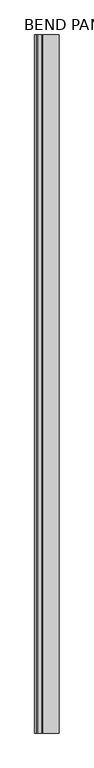
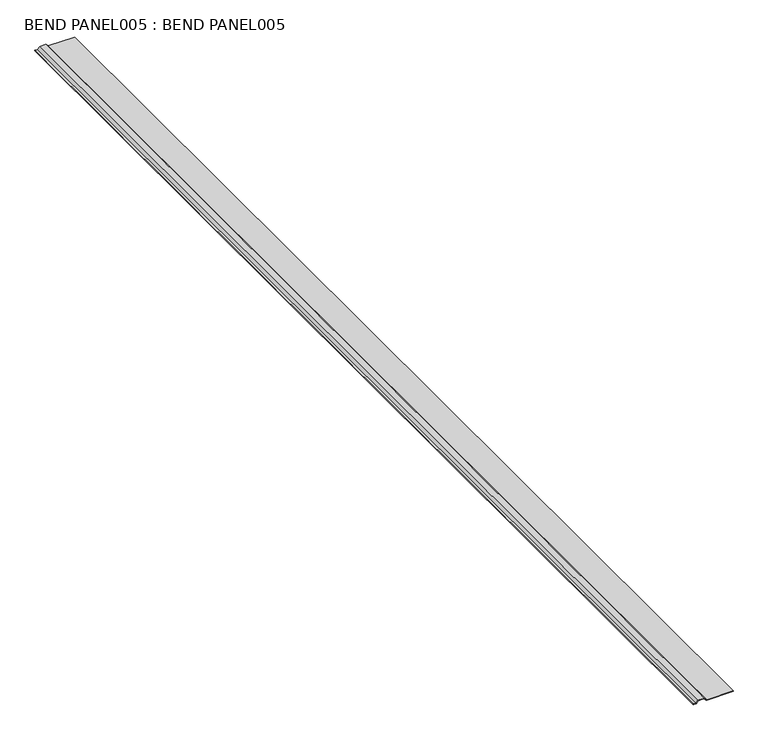
"""IFC4 building model written with IfcOpenShell, lengths in millimetres: proxy geometry, BEND PANEL005 : BEND PANEL005."""

from ifc_helpers import new_model, si_unit, point, frame, frame_2d, origin, place, context, project, spatial, polyline, circle_curve, trimmed, segment, composite_curve, outline, extrude, source, transform, mapped, element, save


def bend_panel005_bend_panel005_8c87a596(model_context):
    return source(origin(), model_context, "Body", "SweptSolid", [
        extrude(outline(composite_curve([segment(polyline([(42575.4212949, 5895.2230694), (42576.6119199, 5895.2230694), (42576.6119199, 5848.7155886), (42580.7948046, 5844.5327039), (42580.7948046, 5833.5642507), (42576.6119199, 5829.381366), (42576.6119199, 5825.5083246), (42575.4212949, 5825.5083246), (42575.4212949, 5829.381366)]), True, "CONTINUOUS"), segment(trimmed(circle_curve(frame_2d((42576.6119199, 5829.381366)), 1.190625), [point((42575.4212949, 5829.381366))], [point((42575.7700209, 5830.223265))], False, "CARTESIAN"), True, "CONTINUOUS"), segment(polyline([(42575.7700209, 5830.223265), (42579.6041796, 5834.0574237), (42579.6041796, 5844.0395308), (42575.7700209, 5847.8736895)]), True, "CONTINUOUS"), segment(trimmed(circle_curve(frame_2d((42576.6119199, 5848.7155885)), 1.190625), [point((42575.7700209, 5847.8736895))], [point((42575.4212949, 5848.7155885))], False, "CARTESIAN"), True, "CONTINUOUS"), segment(polyline([(42575.4212949, 5848.7155885), (42575.4212949, 5895.2230694)]), True, "CONTINUOUS")], self_intersect=False)), frame((0.0, -1052.8906574, 0.0), z_axis=(0.0, 1.0, 0.0), x_axis=(0.0, 0.0, 1.0)), (0.0, 0.0, 1.0), 1999.85),
    ])


if __name__ == "__main__":
    model = new_model("IFC4")
    model_context = context("Model", 3, world=origin())
    ifc_project = project(units=[si_unit("LENGTHUNIT", "METRE", prefix="MILLI")], contexts=[model_context])
    site = spatial("IfcSite", under=ifc_project)
    building = spatial("IfcBuilding", under=site)
    placement = place(None, origin())
    bend_panel005_bend_panel005_shape = bend_panel005_bend_panel005_8c87a596(model_context)
    element("IfcBuildingElementProxy", 1, Name="BEND PANEL005 : BEND PANEL005", ObjectType="BEND PANEL005 : BEND PANEL005", at=placement, inside=building, context=model_context, shape_type="MappedRepresentation", body=[
        mapped(bend_panel005_bend_panel005_shape, transform((0.0, 0.0, 0.0), x_axis=(1.0, 0.0, 0.0), y_axis=(0.0, 1.0, 0.0), z_axis=(0.0, 0.0, 1.0))),
    ])
    save(model, "model.ifc")

# Revit data of these elements
# Type "BEND PANEL005 : BEND PANEL005"
#   NameOverride = "BEND PANEL005"
# Element 1 (IfcBuildingElementProxy, "BEND PANEL005 : BEND PANEL005")
#   Materials on its faces: "METAL PROFILE"
# Materials
#   "METAL PROFILE": class "Unassigned", colour RGB 128 128 128, transparency 0
